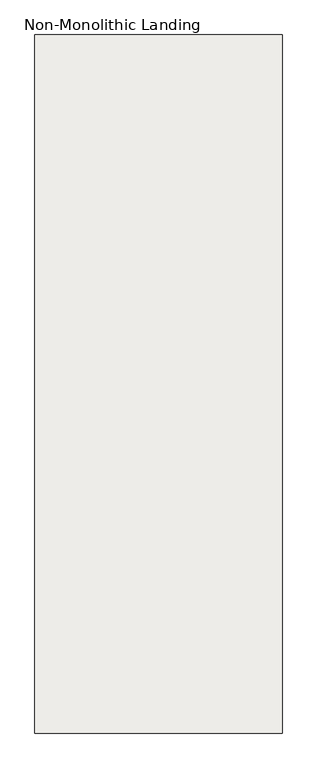
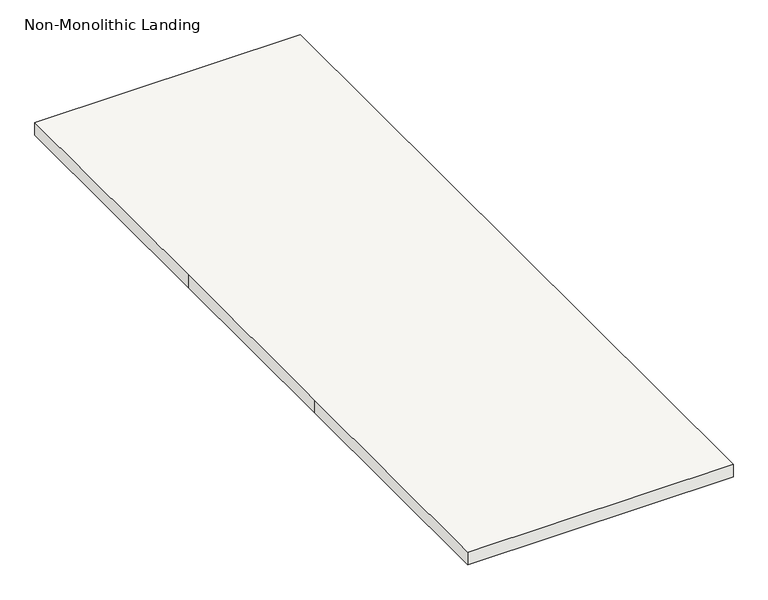
"""IFC4 building model written with IfcOpenShell, lengths in millimetres: slab geometry, Non-Monolithic Landing."""

from ifc_helpers import new_model, si_unit, frame, origin, place, context, project, spatial, polyline, outline, extrude, source, transform, mapped, element, save


def non_monolithic_landing_825fa91f(model_context):
    return source(origin(), model_context, "Body", "SweptSolid", [
        extrude(outline(polyline([(10150.7119026, -2663.8378596), (10150.7119026, -1838.2971943), (10150.7119026, -838.2971943), (11150.7119026, -838.2971943), (11150.7119026, -3663.8378596), (10150.7119026, -3663.8378596), (10150.7119026, -2663.8378596)])), frame((0.0, 0.0, 1714.7058824), z_axis=(0.0, 0.0, 1.0), x_axis=(1.0, 0.0, 0.0)), (0.0, 0.0, 1.0), 50.0),
    ])


if __name__ == "__main__":
    model = new_model("IFC4")
    model_context = context("Model", 3, world=origin())
    ifc_project = project(units=[si_unit("LENGTHUNIT", "METRE", prefix="MILLI")], contexts=[model_context])
    site = spatial("IfcSite", under=ifc_project)
    building = spatial("IfcBuilding", under=site)
    placement = place(None, origin())
    non_monolithic_landing_shape = non_monolithic_landing_825fa91f(model_context)
    element("IfcSlab", 1, ObjectType="Non-Monolithic Landing", at=placement, inside=building, context=model_context, shape_type="MappedRepresentation", body=[
        mapped(non_monolithic_landing_shape, transform((0.0, 0.0, 0.0), x_axis=(1.0, 0.0, 0.0), y_axis=(0.0, 1.0, 0.0), z_axis=(0.0, 0.0, 1.0))),
    ])
    save(model, "model.ifc")
